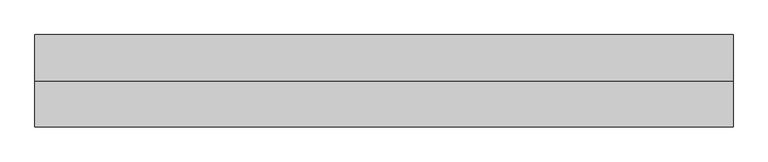
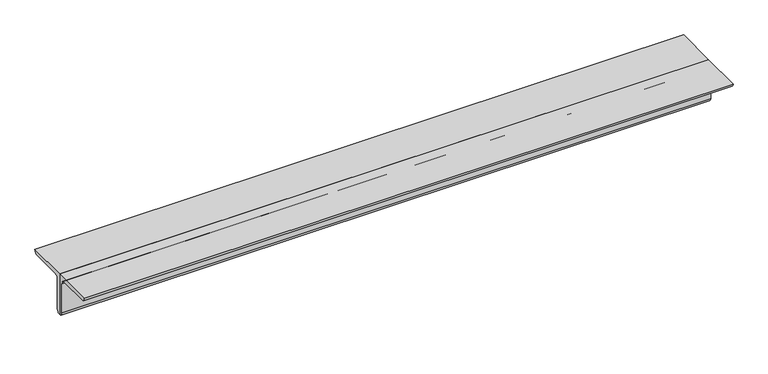
"""IFC4 building model written with IfcOpenShell, lengths in millimetres: member geometry, 0123_Steel Framing_2Ls-KSD3502 : H_SB_AR_S04_2Ls-130x130x12_VBR1."""

from ifc_helpers import new_model, si_unit, point, frame, frame_2d, origin, place, context, project, spatial, polyline, circle_curve, trimmed, segment, composite_curve, outline, extrude, source, transform, mapped, element, save


def member_0ae2001c(model_context):
    return source(origin(), model_context, "Body", "SweptSolid", [
        extrude(outline(composite_curve([segment(polyline([(0.0, 36.4), (130.0, 36.4)]), True, "CONTINUOUS"), segment(trimmed(circle_curve(frame_2d((118.0, 36.4)), 12.0), [point((130.0, 36.4))], [point((118.0, 24.4))], False, "CARTESIAN"), True, "CONTINUOUS"), segment(polyline([(118.0, 24.4), (24.0, 24.4)]), True, "CONTINUOUS"), segment(trimmed(circle_curve(frame_2d((24.0, 12.4)), 12.0), [point((24.0, 24.4))], [point((12.0, 12.4))], True, "CARTESIAN"), True, "CONTINUOUS"), segment(polyline([(12.0, 12.4), (12.0, -81.6)]), True, "CONTINUOUS"), segment(trimmed(circle_curve(frame_2d((0.0, -81.6)), 12.0), [point((12.0, -81.6))], [point((0.0, -93.6))], False, "CARTESIAN"), True, "CONTINUOUS"), segment(polyline([(0.0, -93.6), (0.0, 36.4)]), True, "CONTINUOUS")], self_intersect=False)), frame((-912.8215992, 0.0, 0.0), z_axis=(1.0, 0.0, 0.0), x_axis=(0.0, 1.0, 0.0)), (0.0, 0.0, 1.0), 1965.6424176),
        extrude(outline(composite_curve([segment(polyline([(0.0, 36.4), (0.0, -93.6)]), True, "CONTINUOUS"), segment(trimmed(circle_curve(frame_2d((0.0, -81.6)), 12.0), [point((0.0, -93.6))], [point((-12.0, -81.6))], False, "CARTESIAN"), True, "CONTINUOUS"), segment(polyline([(-12.0, -81.6), (-12.0, 12.4)]), True, "CONTINUOUS"), segment(trimmed(circle_curve(frame_2d((-24.0, 12.4)), 12.0), [point((-12.0, 12.4))], [point((-24.0, 24.4))], True, "CARTESIAN"), True, "CONTINUOUS"), segment(polyline([(-24.0, 24.4), (-118.0, 24.4)]), True, "CONTINUOUS"), segment(trimmed(circle_curve(frame_2d((-118.0, 36.4)), 12.0), [point((-118.0, 24.4))], [point((-130.0, 36.4))], False, "CARTESIAN"), True, "CONTINUOUS"), segment(polyline([(-130.0, 36.4), (0.0, 36.4)]), True, "CONTINUOUS")], self_intersect=False)), frame((-912.8215992, 0.0, 0.0), z_axis=(1.0, 0.0, 0.0), x_axis=(0.0, 1.0, 0.0)), (0.0, 0.0, 1.0), 1965.6424176),
    ])


if __name__ == "__main__":
    model = new_model("IFC4")
    model_context = context("Model", 3, world=origin())
    ifc_project = project(units=[si_unit("LENGTHUNIT", "METRE", prefix="MILLI")], contexts=[model_context])
    site = spatial("IfcSite", under=ifc_project)
    building = spatial("IfcBuilding", under=site)
    placement = place(None, origin())
    member_shape = member_0ae2001c(model_context)
    element("IfcMember", 1, ObjectType="0123_Steel Framing_2Ls-KSD3502 : H_SB_AR_S04_2Ls-130x130x12_VBR1", at=placement, inside=building, context=model_context, shape_type="MappedRepresentation", body=[
        mapped(member_shape, transform((0.0, 0.0, 0.0), x_axis=(1.0, 0.0, 0.0), y_axis=(0.0, 1.0, 0.0), z_axis=(0.0, 0.0, 1.0))),
    ])
    save(model, "model.ifc")

# Revit data of these elements
# Type "0123_Steel Framing_2Ls-KSD3502 : H_SB_AR_S04_2Ls-130x130x12_VBR1"
#   Assembly Code = "B10"
#   Legs = "SLBB"
#   W = 8.97
#   Perimeter = 1.04 m²/m
#   Nominal Weight = 46.80 kgf/m
#   Length [instance default] = 1000 mm
#   Space = 0 mm
#   b = 130 mm
#   d = 130 mm
#   t = 12 mm
#   y = 36.4 mm
#   A = 0.005952 m²
#   Structural Material [instance default] = Steel ASTM A36
# Element 1 (IfcMember, "0123_Steel Framing_2Ls-KSD3502 : H_SB_AR_S04_2Ls-130x130x12_VBR1")
#   Structural Material = Steel, 45-345
#   Materials on its faces: "Steel, 45-345"
# Materials
#   "Steel ASTM A36": class "Metal", colour RGB 199 199 199, transparency 0, Description = "Structural steel, ASTM A36 Grade B, mill finish", Cost = 0
#   "Steel, 45-345": class "Metal", colour RGB 189 187 185, transparency 0, Description = "Steel 345 MPa", Cost = 0
